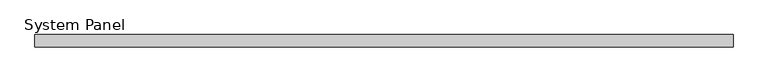
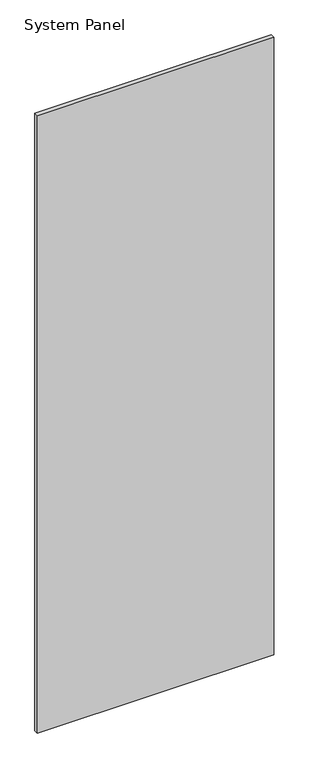
"""IFC4 building model written with IfcOpenShell, lengths in millimetres: plate geometry, System Panel : WWm-Glass-20mm-10mmOffset."""

import ifcopenshell
import ifcopenshell.guid

model = None  # the IFC model being written
_history = None  # IfcOwnerHistory: only IFC2X3 demands one
_inside = {}  # id of a spatial element -> (the spatial element, [elements in it])
_under = {}  # id of a project, library or spatial element -> (it, [spatial elements below it])
_declared = {}  # id of a project -> (the project, [libraries it declares])
_typed = {}  # id of a type object -> (the type object, [elements of that type])
_made_of = {}  # id of a material, layer set ... -> (it, [elements and type objects made of it])


def new_model(schema):
    """Start an empty IFC model of exactly this schema.

    Asked for "IFC4X3", IfcOpenShell would pick the latest addendum, in which some entities
    have other attributes; the version numbers below select the first issue.
    IFC2X3 requires an IfcOwnerHistory on every rooted entity: one is made here for all.
    """
    global model, _history
    if schema == "IFC4X3":
        model = ifcopenshell.file(schema_version=(4, 3, 0, 0))
    else:
        model = ifcopenshell.file(schema=schema)
    _inside.clear()
    _under.clear()
    _declared.clear()
    _typed.clear()
    _made_of.clear()
    _history = None
    if model.schema == "IFC2X3":
        org = make("IfcOrganization", Name="unknown")
        user = make(
            "IfcPersonAndOrganization",
            ThePerson=make("IfcPerson", FamilyName="unknown"),
            TheOrganization=org,
        )
        app = make(
            "IfcApplication",
            ApplicationDeveloper=org,
            Version="unknown",
            ApplicationFullName="unknown",
            ApplicationIdentifier="unknown",
        )
        _history = make(
            "IfcOwnerHistory",
            OwningUser=user,
            OwningApplication=app,
            ChangeAction="ADDED",
            CreationDate=0,
        )
    return model


def make(cls, **values):
    """One entity of the class cls with the attributes given. An attribute that is None is left unset."""
    return model.create_entity(
        cls, **{name: value for name, value in values.items() if value is not None}
    )


def rooted(cls, **values):
    """An entity with a GlobalId (a new one), such as an element, a storey or a relation."""
    return make(cls, GlobalId=ifcopenshell.guid.new(), OwnerHistory=_history, **values)


def si_unit(unit_type, name, prefix=None):
    """IfcSIUnit, for example si_unit("LENGTHUNIT", "METRE", prefix="MILLI")."""
    return make("IfcSIUnit", UnitType=unit_type, Prefix=prefix, Name=name)


def assignment(units):
    """IfcUnitAssignment: the units of a project."""
    return None if units is None else make("IfcUnitAssignment", Units=units)


def point(xyz):
    """IfcCartesianPoint."""
    return None if xyz is None else make("IfcCartesianPoint", Coordinates=xyz)


def direction(xyz):
    """IfcDirection."""
    return None if xyz is None else make("IfcDirection", DirectionRatios=xyz)


def frame(location, z_axis=None, x_axis=None):
    """IfcAxis2Placement3D, a coordinate frame: its origin and axes. An axis left out is left unset."""
    return make(
        "IfcAxis2Placement3D",
        Location=point(location),
        Axis=direction(z_axis),
        RefDirection=direction(x_axis),
    )


def origin():
    """The frame at (0, 0, 0) with its axes left unset."""
    return frame((0.0, 0.0, 0.0))


def origin_with_axes():
    """The frame at (0, 0, 0) with the z axis (0, 0, 1) and the x axis (1, 0, 0) written out."""
    return frame((0.0, 0.0, 0.0), z_axis=(0.0, 0.0, 1.0), x_axis=(1.0, 0.0, 0.0))


def place(relative_to, where):
    """IfcLocalPlacement: puts the frame where relative to a parent placement (None: the world)."""
    return make(
        "IfcLocalPlacement", PlacementRelTo=relative_to, RelativePlacement=where
    )


def context(
    kind, dimensions, precision=None, world=None, true_north=None, identifier=None
):
    """IfcGeometricRepresentationContext, for example the 3D "Model" context."""
    return make(
        "IfcGeometricRepresentationContext",
        ContextIdentifier=identifier,
        ContextType=kind,
        CoordinateSpaceDimension=dimensions,
        Precision=precision,
        WorldCoordinateSystem=world,
        TrueNorth=true_north,
    )


def project(units=None, contexts=None):
    """IfcProject with its units and contexts."""
    return rooted(
        "IfcProject",
        Name="project",
        RepresentationContexts=contexts,
        UnitsInContext=assignment(units),
    )


def spatial(cls, under=None, at=None, **own):
    """A site, building, storey or space (cls), placed at a placement, below another one or the project."""
    s = rooted(cls, ObjectPlacement=at, **own)
    if under is not None:
        _under.setdefault(under.id(), (under, []))[1].append(s)
    return s


def polyline(points):
    """IfcPolyline through the points."""
    return make("IfcPolyline", Points=[point(p) for p in points])


def outline(outer, holes=None, kind="AREA"):
    """IfcArbitraryClosedProfileDef: a profile drawn as a closed curve; with holes, ...WithVoids."""
    if holes is None:
        return make("IfcArbitraryClosedProfileDef", ProfileType=kind, OuterCurve=outer)
    return make(
        "IfcArbitraryProfileDefWithVoids",
        ProfileType=kind,
        OuterCurve=outer,
        InnerCurves=holes,
    )


def extrude(swept, where, along, depth):
    """IfcExtrudedAreaSolid: the profile swept, set in the frame where, extruded along a direction by depth."""
    return make(
        "IfcExtrudedAreaSolid",
        SweptArea=swept,
        Position=where,
        ExtrudedDirection=direction(along),
        Depth=depth,
    )


def shape(context_of_items, identifier, shape_type, items):
    """IfcShapeRepresentation: the items that make up one representation, for example the "Body"."""
    return make(
        "IfcShapeRepresentation",
        ContextOfItems=context_of_items,
        RepresentationIdentifier=identifier,
        RepresentationType=shape_type,
        Items=items,
    )


def source(mapping_origin, context_of_items, identifier, shape_type, items):
    """IfcRepresentationMap: a shape defined once, which mapped items show again and again."""
    return make(
        "IfcRepresentationMap",
        MappingOrigin=mapping_origin,
        MappedRepresentation=shape(context_of_items, identifier, shape_type, items),
    )


def transform(
    local_origin,
    x_axis=None,
    y_axis=None,
    z_axis=None,
    scale=None,
    scale2=None,
    scale3=None,
    uniform=True,
):
    """IfcCartesianTransformationOperator3D, or its non-uniform kind. x_axis, y_axis, z_axis: its Axis1, 2, 3."""
    if uniform:
        return make(
            "IfcCartesianTransformationOperator3D",
            Axis1=direction(x_axis),
            Axis2=direction(y_axis),
            LocalOrigin=point(local_origin),
            Scale=scale,
            Axis3=direction(z_axis),
        )
    return make(
        "IfcCartesianTransformationOperator3DnonUniform",
        Axis1=direction(x_axis),
        Axis2=direction(y_axis),
        LocalOrigin=point(local_origin),
        Scale=scale,
        Axis3=direction(z_axis),
        Scale2=scale2,
        Scale3=scale3,
    )


def mapped(mapping_source, mapping_target):
    """IfcMappedItem: shows the shape of a source again, moved by a transform."""
    return make(
        "IfcMappedItem", MappingSource=mapping_source, MappingTarget=mapping_target
    )


def made_of(thing, what):
    """Note that an element or type object is made of a material, layer set ...; save() writes the relation."""
    if what is not None:
        _made_of.setdefault(what.id(), (what, []))[1].append(thing)
    return thing


def element(
    cls,
    number,
    at=None,
    inside=None,
    cuts=None,
    type_object=None,
    material=None,
    context=None,
    identifier="Body",
    shape_type=None,
    held_by="IfcProductDefinitionShape",
    body=None,
    shapes=None,
    **own,
):
    """One element of the class cls, such as IfcWall. Its Tag is "e" and its number.

    at: its placement. inside: the storey or other place that contains it. cuts: it is an
    opening in that element (IfcRelVoidsElement). A single representation is given by context,
    identifier, shape_type and body (its items); several are given by shapes. held_by: the class
    of the entity that holds the representations. save() writes the other relations.
    """
    e = rooted(cls, Tag="e%d" % number, ObjectPlacement=at, **own)
    if body is not None:
        shapes = [shape(context, identifier, shape_type, body)]
    if shapes is not None:
        e.Representation = make(held_by, Representations=shapes)
    if inside is not None:
        _inside.setdefault(inside.id(), (inside, []))[1].append(e)
    if cuts is not None:
        rooted(
            "IfcRelVoidsElement", RelatingBuildingElement=cuts, RelatedOpeningElement=e
        )
    if type_object is not None:
        _typed.setdefault(type_object.id(), (type_object, []))[1].append(e)
    return made_of(e, material)


def aggregate(whole, parts):
    """IfcRelAggregates: a whole, such as a stair, and the parts it consists of."""
    return rooted("IfcRelAggregates", RelatingObject=whole, RelatedObjects=parts)


def save(model, path):
    """Write the relations noted so far, then the file.

    IfcRelAggregates (storeys below a building ...), IfcRelContainedInSpatialStructure (elements
    in a storey), IfcRelDefinesByType, IfcRelAssociatesMaterial and IfcRelDeclares: one each for
    every whole, place, type object, material and project.
    """
    for whole, parts in _under.values():
        aggregate(whole, parts)
    for where, things in _inside.values():
        rooted(
            "IfcRelContainedInSpatialStructure",
            RelatedElements=things,
            RelatingStructure=where,
        )
    for kind, things in _typed.values():
        rooted("IfcRelDefinesByType", RelatedObjects=things, RelatingType=kind)
    for what, things in _made_of.values():
        rooted("IfcRelAssociatesMaterial", RelatedObjects=things, RelatingMaterial=what)
    for by, libraries in _declared.values():
        rooted("IfcRelDeclares", RelatingContext=by, RelatedDefinitions=libraries)
    model.write(path)


def system_panel_b181fc9a(model_context):
    return source(origin(), model_context, "Body", "SweptSolid", [
        extrude(outline(polyline([(570.5171322, 0.0), (-570.5171322, 0.0), (-570.5171322, 20.0), (570.5171322, 20.0), (570.5171322, 0.0)])), origin_with_axes(), (0.0, 0.0, 1.0), 3150.0),
    ])


if __name__ == "__main__":
    model = new_model("IFC4")
    model_context = context("Model", 3, world=origin())
    ifc_project = project(units=[si_unit("LENGTHUNIT", "METRE", prefix="MILLI")], contexts=[model_context])
    site = spatial("IfcSite", under=ifc_project)
    building = spatial("IfcBuilding", under=site)
    placement = place(None, origin())
    system_panel_shape = system_panel_b181fc9a(model_context)
    element("IfcPlate", 1, ObjectType="System Panel : WWm-Glass-20mm-10mmOffset", at=placement, inside=building, context=model_context, shape_type="MappedRepresentation", body=[
        mapped(system_panel_shape, transform((0.0, 0.0, 0.0), x_axis=(1.0, 0.0, 0.0), y_axis=(0.0, 1.0, 0.0), z_axis=(0.0, 0.0, 1.0))),
    ])
    save(model, "model.ifc")

# Revit data of these elements
# Type "System Panel : WWm-Glass-20mm-10mmOffset"
#   Finish = ""
# Element 1 (IfcPlate, "System Panel : WWm-Glass-20mm-10mmOffset")
#   Materials on its faces: "WW-EC-GL-Storefront"
# Materials
#   "WW-EC-GL-Storefront": class "Glass", colour RGB 236 240 239, transparency 0.85, Description = "Storefront Glass", Cost = 0
